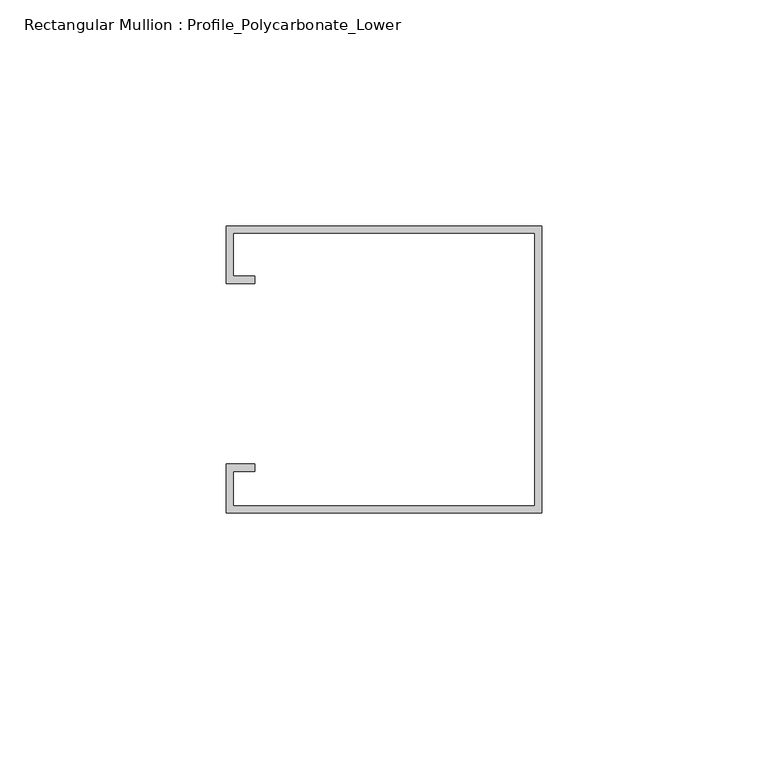
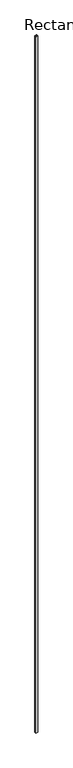
"""IFC4 building model written with IfcOpenShell, lengths in millimetres: member geometry, Rectangular Mullion : Profile_Polycarbonate_Lower."""

from ifc_helpers import new_model, si_unit, frame, origin, place, context, project, spatial, polyline, outline, extrude, source, transform, mapped, element, save


def rectangular_mullion_profile_polycarbonate_lower_8f34c2a7(model_context):
    return source(origin(), model_context, "Body", "SweptSolid", [
        extrude(outline(polyline([(0.0, 32.7), (0.0, -30.8), (-69.85, -30.8), (-69.85, -20.0), (-63.5, -20.0), (-63.5, -21.5875), (-68.2625, -21.5875), (-68.2625, -29.2125), (-1.5875, -29.2125), (-1.5875, 31.1125), (-68.2625, 31.1125), (-68.2625, 21.5875), (-63.5, 21.5875), (-63.5, 20.0), (-69.85, 20.0), (-69.85, 32.7), (0.0, 32.7)])), frame((0.0, 0.0, -25395.2375), z_axis=(0.0, 0.0, 1.0), x_axis=(1.0, 0.0, 0.0)), (0.0, 0.0, 1.0), 25395.2375),
    ])


if __name__ == "__main__":
    model = new_model("IFC4")
    model_context = context("Model", 3, world=origin())
    ifc_project = project(units=[si_unit("LENGTHUNIT", "METRE", prefix="MILLI")], contexts=[model_context])
    site = spatial("IfcSite", under=ifc_project)
    building = spatial("IfcBuilding", under=site)
    placement = place(None, origin())
    rectangular_mullion_profile_polycarbonate_lower_shape = rectangular_mullion_profile_polycarbonate_lower_8f34c2a7(model_context)
    element("IfcMember", 1, ObjectType="Rectangular Mullion : Profile_Polycarbonate_Lower", at=placement, inside=building, context=model_context, shape_type="MappedRepresentation", body=[
        mapped(rectangular_mullion_profile_polycarbonate_lower_shape, transform((0.0, 0.0, 0.0), x_axis=(1.0, 0.0, 0.0), y_axis=(0.0, 1.0, 0.0), z_axis=(0.0, 0.0, 1.0))),
    ])
    save(model, "model.ifc")

# Revit data of these elements
# Type "Rectangular Mullion : Profile_Polycarbonate_Lower"
#   built-in parameter 1007322 = 0.208333 (stored number, unit not read)
#   built-in parameter 1007321 = 0 (stored number, unit not read)
#   built-in parameter 1007320 = 0.00520833 (stored number, unit not read)
# Element 1 (IfcMember, "Rectangular Mullion : Profile_Polycarbonate_Lower")
#   Materials on its faces: "ALUMINUM PROFILE AT POLYCARBONATE PANEL"
# Materials
#   "ALUMINUM PROFILE AT POLYCARBONATE PANEL": class "Metal", colour RGB 244 244 244, transparency 0, Description = "Aluminum 6061", Cost = 0
